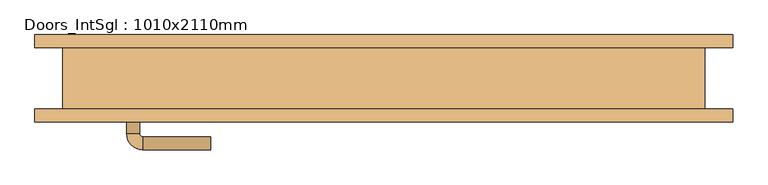
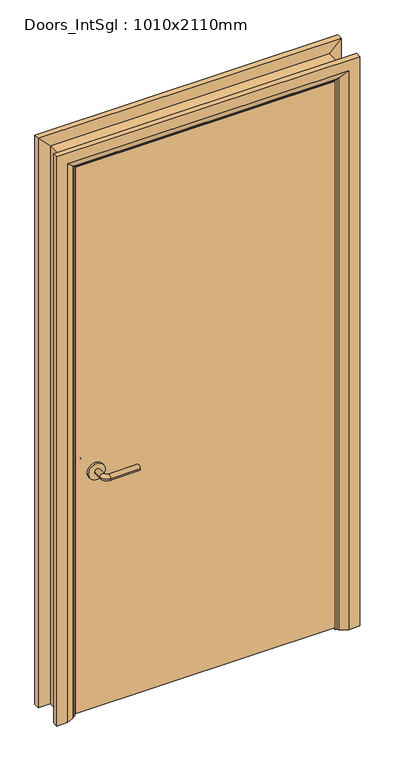
"""IFC4 building model written with IfcOpenShell, lengths in millimetres: door geometry, Doors_IntSgl : 1010x2110mm."""

import ifcopenshell
import ifcopenshell.guid

model = None  # the IFC model being written
_history = None  # IfcOwnerHistory: only IFC2X3 demands one
_inside = {}  # id of a spatial element -> (the spatial element, [elements in it])
_under = {}  # id of a project, library or spatial element -> (it, [spatial elements below it])
_declared = {}  # id of a project -> (the project, [libraries it declares])
_typed = {}  # id of a type object -> (the type object, [elements of that type])
_made_of = {}  # id of a material, layer set ... -> (it, [elements and type objects made of it])


def new_model(schema):
    """Start an empty IFC model of exactly this schema.

    Asked for "IFC4X3", IfcOpenShell would pick the latest addendum, in which some entities
    have other attributes; the version numbers below select the first issue.
    IFC2X3 requires an IfcOwnerHistory on every rooted entity: one is made here for all.
    """
    global model, _history
    if schema == "IFC4X3":
        model = ifcopenshell.file(schema_version=(4, 3, 0, 0))
    else:
        model = ifcopenshell.file(schema=schema)
    _inside.clear()
    _under.clear()
    _declared.clear()
    _typed.clear()
    _made_of.clear()
    _history = None
    if model.schema == "IFC2X3":
        org = make("IfcOrganization", Name="unknown")
        user = make(
            "IfcPersonAndOrganization",
            ThePerson=make("IfcPerson", FamilyName="unknown"),
            TheOrganization=org,
        )
        app = make(
            "IfcApplication",
            ApplicationDeveloper=org,
            Version="unknown",
            ApplicationFullName="unknown",
            ApplicationIdentifier="unknown",
        )
        _history = make(
            "IfcOwnerHistory",
            OwningUser=user,
            OwningApplication=app,
            ChangeAction="ADDED",
            CreationDate=0,
        )
    return model


def make(cls, **values):
    """One entity of the class cls with the attributes given. An attribute that is None is left unset."""
    return model.create_entity(
        cls, **{name: value for name, value in values.items() if value is not None}
    )


def rooted(cls, **values):
    """An entity with a GlobalId (a new one), such as an element, a storey or a relation."""
    return make(cls, GlobalId=ifcopenshell.guid.new(), OwnerHistory=_history, **values)


def si_unit(unit_type, name, prefix=None):
    """IfcSIUnit, for example si_unit("LENGTHUNIT", "METRE", prefix="MILLI")."""
    return make("IfcSIUnit", UnitType=unit_type, Prefix=prefix, Name=name)


def assignment(units):
    """IfcUnitAssignment: the units of a project."""
    return None if units is None else make("IfcUnitAssignment", Units=units)


def point(xyz):
    """IfcCartesianPoint."""
    return None if xyz is None else make("IfcCartesianPoint", Coordinates=xyz)


def direction(xyz):
    """IfcDirection."""
    return None if xyz is None else make("IfcDirection", DirectionRatios=xyz)


def frame(location, z_axis=None, x_axis=None):
    """IfcAxis2Placement3D, a coordinate frame: its origin and axes. An axis left out is left unset."""
    return make(
        "IfcAxis2Placement3D",
        Location=point(location),
        Axis=direction(z_axis),
        RefDirection=direction(x_axis),
    )


def frame_2d(location, x_axis=None):
    """IfcAxis2Placement2D, a coordinate frame in the plane: its origin and x axis."""
    return make(
        "IfcAxis2Placement2D", Location=point(location), RefDirection=direction(x_axis)
    )


def origin():
    """The frame at (0, 0, 0) with its axes left unset."""
    return frame((0.0, 0.0, 0.0))


def place(relative_to, where):
    """IfcLocalPlacement: puts the frame where relative to a parent placement (None: the world)."""
    return make(
        "IfcLocalPlacement", PlacementRelTo=relative_to, RelativePlacement=where
    )


def context(
    kind, dimensions, precision=None, world=None, true_north=None, identifier=None
):
    """IfcGeometricRepresentationContext, for example the 3D "Model" context."""
    return make(
        "IfcGeometricRepresentationContext",
        ContextIdentifier=identifier,
        ContextType=kind,
        CoordinateSpaceDimension=dimensions,
        Precision=precision,
        WorldCoordinateSystem=world,
        TrueNorth=true_north,
    )


def project(units=None, contexts=None):
    """IfcProject with its units and contexts."""
    return rooted(
        "IfcProject",
        Name="project",
        RepresentationContexts=contexts,
        UnitsInContext=assignment(units),
    )


def spatial(cls, under=None, at=None, **own):
    """A site, building, storey or space (cls), placed at a placement, below another one or the project."""
    s = rooted(cls, ObjectPlacement=at, **own)
    if under is not None:
        _under.setdefault(under.id(), (under, []))[1].append(s)
    return s


def polyline(points):
    """IfcPolyline through the points."""
    return make("IfcPolyline", Points=[point(p) for p in points])


def circle_curve(where, radius):
    """IfcCircle in the frame where."""
    return make("IfcCircle", Position=where, Radius=radius)


def ellipse_curve(where, semi_axis1, semi_axis2):
    """IfcEllipse in the frame where."""
    return make(
        "IfcEllipse", Position=where, SemiAxis1=semi_axis1, SemiAxis2=semi_axis2
    )


def trimmed(basis, trim1, trim2, sense, master):
    """IfcTrimmedCurve: the piece of a basis curve between two trims."""
    return make(
        "IfcTrimmedCurve",
        BasisCurve=basis,
        Trim1=trim1,
        Trim2=trim2,
        SenseAgreement=sense,
        MasterRepresentation=master,
    )


def segment(curve, same_sense, transition):
    """IfcCompositeCurveSegment."""
    return make(
        "IfcCompositeCurveSegment",
        Transition=transition,
        SameSense=same_sense,
        ParentCurve=curve,
    )


def composite_curve(segments, self_intersect=None):
    """IfcCompositeCurve: segments joined end to end."""
    return make("IfcCompositeCurve", Segments=segments, SelfIntersect=self_intersect)


def outline(outer, holes=None, kind="AREA"):
    """IfcArbitraryClosedProfileDef: a profile drawn as a closed curve; with holes, ...WithVoids."""
    if holes is None:
        return make("IfcArbitraryClosedProfileDef", ProfileType=kind, OuterCurve=outer)
    return make(
        "IfcArbitraryProfileDefWithVoids",
        ProfileType=kind,
        OuterCurve=outer,
        InnerCurves=holes,
    )


def extrude(swept, where, along, depth):
    """IfcExtrudedAreaSolid: the profile swept, set in the frame where, extruded along a direction by depth."""
    return make(
        "IfcExtrudedAreaSolid",
        SweptArea=swept,
        Position=where,
        ExtrudedDirection=direction(along),
        Depth=depth,
    )


def faces_of(points, faces, orient=None, outer=None):
    """IfcFace entities. A face is a list of loops; a loop is a list of indices into points, from 0.

    orient and outer hold one flag for each loop. By default every Orientation is true, the
    first loop of a face is its IfcFaceOuterBound and the others are IfcFaceBound.
    """
    made = []
    for i, loops in enumerate(faces):
        bounds = []
        for j, loop in enumerate(loops):
            is_outer = j == 0 if outer is None else outer[i][j]
            bounds.append(
                make(
                    "IfcFaceOuterBound" if is_outer else "IfcFaceBound",
                    Bound=make("IfcPolyLoop", Polygon=[points[k] for k in loop]),
                    Orientation=True if orient is None else orient[i][j],
                )
            )
        made.append(make("IfcFace", Bounds=bounds))
    return made


def faceted_brep(points, faces, orient=None, outer=None, voids=None):
    """IfcFacetedBrep: a solid bounded by flat faces; with voids (closed shells), ...WithVoids."""
    shared = [point(p) for p in points]
    hull = make("IfcClosedShell", CfsFaces=faces_of(shared, faces, orient, outer))
    if voids is None:
        return make("IfcFacetedBrep", Outer=hull)
    return make(
        "IfcFacetedBrepWithVoids",
        Outer=hull,
        Voids=[
            make(cls, CfsFaces=faces_of(shared, fs, o, b)) for cls, fs, o, b in voids
        ],
    )


def shape(context_of_items, identifier, shape_type, items):
    """IfcShapeRepresentation: the items that make up one representation, for example the "Body"."""
    return make(
        "IfcShapeRepresentation",
        ContextOfItems=context_of_items,
        RepresentationIdentifier=identifier,
        RepresentationType=shape_type,
        Items=items,
    )


def source(mapping_origin, context_of_items, identifier, shape_type, items):
    """IfcRepresentationMap: a shape defined once, which mapped items show again and again."""
    return make(
        "IfcRepresentationMap",
        MappingOrigin=mapping_origin,
        MappedRepresentation=shape(context_of_items, identifier, shape_type, items),
    )


def transform(
    local_origin,
    x_axis=None,
    y_axis=None,
    z_axis=None,
    scale=None,
    scale2=None,
    scale3=None,
    uniform=True,
):
    """IfcCartesianTransformationOperator3D, or its non-uniform kind. x_axis, y_axis, z_axis: its Axis1, 2, 3."""
    if uniform:
        return make(
            "IfcCartesianTransformationOperator3D",
            Axis1=direction(x_axis),
            Axis2=direction(y_axis),
            LocalOrigin=point(local_origin),
            Scale=scale,
            Axis3=direction(z_axis),
        )
    return make(
        "IfcCartesianTransformationOperator3DnonUniform",
        Axis1=direction(x_axis),
        Axis2=direction(y_axis),
        LocalOrigin=point(local_origin),
        Scale=scale,
        Axis3=direction(z_axis),
        Scale2=scale2,
        Scale3=scale3,
    )


def mapped(mapping_source, mapping_target):
    """IfcMappedItem: shows the shape of a source again, moved by a transform."""
    return make(
        "IfcMappedItem", MappingSource=mapping_source, MappingTarget=mapping_target
    )


def made_of(thing, what):
    """Note that an element or type object is made of a material, layer set ...; save() writes the relation."""
    if what is not None:
        _made_of.setdefault(what.id(), (what, []))[1].append(thing)
    return thing


def element(
    cls,
    number,
    at=None,
    inside=None,
    cuts=None,
    type_object=None,
    material=None,
    context=None,
    identifier="Body",
    shape_type=None,
    held_by="IfcProductDefinitionShape",
    body=None,
    shapes=None,
    **own,
):
    """One element of the class cls, such as IfcWall. Its Tag is "e" and its number.

    at: its placement. inside: the storey or other place that contains it. cuts: it is an
    opening in that element (IfcRelVoidsElement). A single representation is given by context,
    identifier, shape_type and body (its items); several are given by shapes. held_by: the class
    of the entity that holds the representations. save() writes the other relations.
    """
    e = rooted(cls, Tag="e%d" % number, ObjectPlacement=at, **own)
    if body is not None:
        shapes = [shape(context, identifier, shape_type, body)]
    if shapes is not None:
        e.Representation = make(held_by, Representations=shapes)
    if inside is not None:
        _inside.setdefault(inside.id(), (inside, []))[1].append(e)
    if cuts is not None:
        rooted(
            "IfcRelVoidsElement", RelatingBuildingElement=cuts, RelatedOpeningElement=e
        )
    if type_object is not None:
        _typed.setdefault(type_object.id(), (type_object, []))[1].append(e)
    return made_of(e, material)


def aggregate(whole, parts):
    """IfcRelAggregates: a whole, such as a stair, and the parts it consists of."""
    return rooted("IfcRelAggregates", RelatingObject=whole, RelatedObjects=parts)


def save(model, path):
    """Write the relations noted so far, then the file.

    IfcRelAggregates (storeys below a building ...), IfcRelContainedInSpatialStructure (elements
    in a storey), IfcRelDefinesByType, IfcRelAssociatesMaterial and IfcRelDeclares: one each for
    every whole, place, type object, material and project.
    """
    for whole, parts in _under.values():
        aggregate(whole, parts)
    for where, things in _inside.values():
        rooted(
            "IfcRelContainedInSpatialStructure",
            RelatedElements=things,
            RelatingStructure=where,
        )
    for kind, things in _typed.values():
        rooted("IfcRelDefinesByType", RelatedObjects=things, RelatingType=kind)
    for what, things in _made_of.values():
        rooted("IfcRelAssociatesMaterial", RelatedObjects=things, RelatingMaterial=what)
    for by, libraries in _declared.values():
        rooted("IfcRelDeclares", RelatingContext=by, RelatedDefinitions=libraries)
    model.write(path)


def plane_surface(at):
    """IfcPlane: the flat surface through the origin of the frame at, square to its z axis."""
    return make("IfcPlane", Position=at)


def cylinder_surface(at, radius):
    """IfcCylindricalSurface: all points at the distance radius from the z axis of the frame at."""
    return make("IfcCylindricalSurface", Position=at, Radius=radius)


def revolved_surface(curve, axis_point, axis_direction):
    """IfcSurfaceOfRevolution: the curve turned about the line through axis_point along axis_direction."""
    return make(
        "IfcSurfaceOfRevolution",
        SweptCurve=make("IfcArbitraryOpenProfileDef", ProfileType="CURVE", Curve=curve),
        AxisPosition=make("IfcAxis1Placement", Location=point(axis_point), Axis=direction(axis_direction)),
    )


def advanced_brep(points, edges, surfaces, faces):
    """IfcAdvancedBrep: a solid bounded by faces that lie on surfaces and meet in shared edges.

    An edge is (start, end): straight between two places in points (the first is 0);
    or (start, end, curve); or (start, end, curve, False) where it runs against its curve.
    A face is (place in surfaces, loops), or (place, loops, False) where it looks against
    its surface's normal. A loop lists edges by number (the first is 1), with a minus sign
    where the edge is run from its end to its start. The first loop is the outer one.
    """
    corners = [point(p) for p in points]
    vertices = [make("IfcVertexPoint", VertexGeometry=c) for c in corners]
    made = []
    for start, end, *more in edges:
        made.append(
            make(
                "IfcEdgeCurve",
                EdgeStart=vertices[start],
                EdgeEnd=vertices[end],
                EdgeGeometry=more[0] if more else make("IfcPolyline", Points=[corners[start], corners[end]]),
                SameSense=more[1] if len(more) > 1 else True,
            )
        )
    hull = []
    for where, loops, *sense in faces:
        bounds = []
        for j, loop in enumerate(loops):
            ring = [make("IfcOrientedEdge", EdgeElement=made[abs(k) - 1], Orientation=k > 0) for k in loop]
            bounds.append(
                make(
                    "IfcFaceOuterBound" if j == 0 else "IfcFaceBound",
                    Bound=make("IfcEdgeLoop", EdgeList=ring),
                    Orientation=True,
                )
            )
        hull.append(make("IfcAdvancedFace", Bounds=bounds, FaceSurface=surfaces[where], SameSense=sense[0] if sense else True))
    return make("IfcAdvancedBrep", Outer=make("IfcClosedShell", CfsFaces=hull))


def doors_intsgl_1010x2110mm_25c8a350(model_context):
    return source(origin(), model_context, "Body", "SolidModel", [
        advanced_brep(
        [(-398.0, -1.5, 900.0), (-378.0, -1.5, 900.0), (-398.0, 28.5, 900.0), (-378.0, 28.5, 900.0), (-373.0, 33.5, 900.0), (-373.0, 53.5, 900.0), (-268.0, 53.5, 900.0), (-268.0, 33.5, 900.0)],
        [
            (0, 1, circle_curve(frame((-388.0, -1.5, 900.0), z_axis=(0.0, -1.0, 0.0), x_axis=(1.0, 0.0, 0.0)), 10.0)),
            (1, 0, circle_curve(frame((-388.0, -1.5, 900.0), z_axis=(0.0, -1.0, 0.0), x_axis=(1.0, 0.0, 0.0)), 10.0)),
            (0, 2),
            (2, 3, circle_curve(frame((-388.0, 28.5, 900.0), z_axis=(0.0, -1.0, 0.0), x_axis=(1.0, 0.0, 0.0)), 10.0)),
            (3, 1),
            (3, 2, circle_curve(frame((-388.0, 28.5, 900.0), z_axis=(0.0, -1.0, 0.0), x_axis=(1.0, 0.0, 0.0)), 10.0)),
            (4, 3, circle_curve(frame((-373.0, 28.5, 900.0), z_axis=(0.0, 0.0, 1.0), x_axis=(-1.0, 0.0, 0.0)), 5.0)),
            (2, 5, circle_curve(frame((-373.0, 28.5, 900.0), z_axis=(0.0, 0.0, -1.0), x_axis=(-1.0, 0.0, 0.0)), 25.0)),
            (5, 4, circle_curve(frame((-373.0, 43.5, 900.0), z_axis=(-1.0, 0.0, 0.0), x_axis=(0.0, -1.0, 0.0)), 10.0)),
            (4, 5, circle_curve(frame((-373.0, 43.5, 900.0), z_axis=(-1.0, 0.0, 0.0), x_axis=(0.0, -1.0, 0.0)), 10.0)),
            (6, 7, circle_curve(frame((-268.0, 43.5, 900.0), z_axis=(1.0, 0.0, 0.0), x_axis=(0.0, -1.0, 0.0)), 10.0)),
            (7, 6, circle_curve(frame((-268.0, 43.5, 900.0), z_axis=(1.0, 0.0, 0.0), x_axis=(0.0, -1.0, 0.0)), 10.0)),
            (5, 6),
            (7, 4),
        ],
        [
            plane_surface(frame((-388.0, -1.5, 900.0), z_axis=(0.0, -1.0, 0.0), x_axis=(0.0, 0.0, 1.0))),
            cylinder_surface(frame((-388.0, -1.5, 900.0), z_axis=(0.0, -1.0, 0.0), x_axis=(1.0, 0.0, 0.0)), 10.0),
            revolved_surface(trimmed(ellipse_curve(frame((-388.0, 28.5, 900.0), z_axis=(0.0, -1.0, 0.0), x_axis=(1.0, 0.0, 0.0)), 10.0, 10.0), [point((-398.0, 28.5, 900.0))], [point((-378.0, 28.5, 900.0))], True, "CARTESIAN"), (-373.0, 28.5, 900.0), (0.0, 0.0, -1.0)),
            revolved_surface(trimmed(ellipse_curve(frame((-388.0, 28.5, 900.0), z_axis=(0.0, -1.0, 0.0), x_axis=(1.0, 0.0, 0.0)), 10.0, 10.0), [point((-378.0, 28.5, 900.0))], [point((-398.0, 28.5, 900.0))], True, "CARTESIAN"), (-373.0, 28.5, 900.0), (0.0, 0.0, -1.0)),
            plane_surface(frame((-268.0, 43.5, 900.0), z_axis=(1.0, 0.0, 0.0), x_axis=(0.0, 0.0, 1.0))),
            cylinder_surface(frame((-373.0, 43.5, 900.0), z_axis=(-1.0, 0.0, 0.0), x_axis=(0.0, -1.0, 0.0)), 10.0),
        ],
        [
            (0, [[1, 2]]),
            (1, [[-1, 3, 4, 5]]),
            (1, [[-2, -5, 6, -3]]),
            (2, [[7, -4, 8, 9]]),
            (3, [[-8, -6, -7, 10]]),
            (4, [[11, 12]]),
            (5, [[-9, 13, -12, 14]]),
            (5, [[-10, -14, -11, -13]]),
        ],
    ),
        extrude(outline(composite_curve([segment(trimmed(circle_curve(frame_2d((900.0, -390.5)), 30.0), [point((900.0, -420.5))], [point((900.0, -360.5))], False, "CARTESIAN"), True, "CONTINUOUS"), segment(trimmed(circle_curve(frame_2d((900.0, -390.5)), 30.0), [point((900.0, -360.5))], [point((900.0, -420.5))], False, "CARTESIAN"), True, "CONTINUOUS")], self_intersect=False)), frame((0.0, -9.5, 0.0), z_axis=(0.0, 1.0, 0.0), x_axis=(0.0, 0.0, 1.0)), (0.0, 0.0, 1.0), 8.0),
        advanced_brep(
        [(-398.0, -55.5, 900.0), (-378.0, -55.5, 900.0), (-378.0, -85.5, 900.0), (-398.0, -85.5, 900.0), (-373.0, -90.5, 900.0), (-373.0, -110.5, 900.0), (-268.0, -110.5, 900.0), (-268.0, -90.5, 900.0)],
        [
            (0, 1, circle_curve(frame((-388.0, -55.5, 900.0), z_axis=(0.0, 1.0, 0.0), x_axis=(1.0, 0.0, 0.0)), 10.0)),
            (1, 0, circle_curve(frame((-388.0, -55.5, 900.0), z_axis=(0.0, 1.0, 0.0), x_axis=(1.0, 0.0, 0.0)), 10.0)),
            (1, 2),
            (2, 3, circle_curve(frame((-388.0, -85.5, 900.0), z_axis=(0.0, 1.0, 0.0), x_axis=(1.0, 0.0, 0.0)), 10.0)),
            (3, 0),
            (3, 2, circle_curve(frame((-388.0, -85.5, 900.0), z_axis=(0.0, 1.0, 0.0), x_axis=(1.0, 0.0, 0.0)), 10.0)),
            (4, 5, circle_curve(frame((-373.0, -100.5, 900.0), z_axis=(-1.0, 0.0, 0.0), x_axis=(0.0, 1.0, 0.0)), 10.0)),
            (5, 3, circle_curve(frame((-373.0, -85.5, 900.0), z_axis=(0.0, 0.0, -1.0), x_axis=(-1.0, 0.0, 0.0)), 25.0)),
            (2, 4, circle_curve(frame((-373.0, -85.5, 900.0), z_axis=(0.0, 0.0, 1.0), x_axis=(-1.0, 0.0, 0.0)), 5.0)),
            (5, 4, circle_curve(frame((-373.0, -100.5, 900.0), z_axis=(-1.0, 0.0, 0.0), x_axis=(0.0, 1.0, 0.0)), 10.0)),
            (6, 7, circle_curve(frame((-268.0, -100.5, 900.0), z_axis=(1.0, 0.0, 0.0), x_axis=(0.0, 1.0, 0.0)), 10.0)),
            (7, 6, circle_curve(frame((-268.0, -100.5, 900.0), z_axis=(1.0, 0.0, 0.0), x_axis=(0.0, 1.0, 0.0)), 10.0)),
            (4, 7),
            (6, 5),
        ],
        [
            plane_surface(frame((-388.0, -55.5, 900.0), z_axis=(0.0, 1.0, 0.0), x_axis=(0.0, 0.0, 1.0))),
            cylinder_surface(frame((-388.0, -55.5, 900.0), z_axis=(0.0, 1.0, 0.0), x_axis=(1.0, 0.0, 0.0)), 10.0),
            revolved_surface(trimmed(ellipse_curve(frame((-388.0, -85.5, 900.0), z_axis=(0.0, -1.0, 0.0), x_axis=(1.0, 0.0, 0.0)), 10.0, 10.0), [point((-398.0, -85.5, 900.0))], [point((-378.0, -85.5, 900.0))], True, "CARTESIAN"), (-373.0, -85.5, 900.0), (0.0, 0.0, -1.0)),
            revolved_surface(trimmed(ellipse_curve(frame((-388.0, -85.5, 900.0), z_axis=(0.0, -1.0, 0.0), x_axis=(1.0, 0.0, 0.0)), 10.0, 10.0), [point((-378.0, -85.5, 900.0))], [point((-398.0, -85.5, 900.0))], True, "CARTESIAN"), (-373.0, -85.5, 900.0), (0.0, 0.0, -1.0)),
            plane_surface(frame((-268.0, -100.5, 900.0), z_axis=(1.0, 0.0, 0.0), x_axis=(0.0, 0.0, 1.0))),
            cylinder_surface(frame((-373.0, -100.5, 900.0), z_axis=(-1.0, 0.0, 0.0), x_axis=(0.0, 1.0, 0.0)), 10.0),
        ],
        [
            (0, [[1, 2]]),
            (1, [[3, 4, 5, -2]]),
            (1, [[-5, 6, -3, -1]]),
            (2, [[7, 8, -4, 9]]),
            (3, [[10, -9, -6, -8]]),
            (4, [[11, 12]]),
            (5, [[13, -11, 14, -7]]),
            (5, [[-14, -12, -13, -10]]),
        ],
    ),
        extrude(outline(composite_curve([segment(trimmed(circle_curve(frame_2d((900.0, -390.5)), 30.0), [point((900.0, -420.5))], [point((900.0, -360.5))], False, "CARTESIAN"), True, "CONTINUOUS"), segment(trimmed(circle_curve(frame_2d((900.0, -390.5)), 30.0), [point((900.0, -360.5))], [point((900.0, -420.5))], False, "CARTESIAN"), True, "CONTINUOUS")], self_intersect=False)), frame((0.0, -55.5, 0.0), z_axis=(0.0, 1.0, 0.0), x_axis=(0.0, 0.0, 1.0)), (0.0, 0.0, 1.0), 8.0),
        extrude(outline(polyline([(463.0, -9.5), (463.0, -47.5), (-463.0, -47.5), (-463.0, -9.5), (463.0, -9.5)])), frame((0.0, 0.0, 8.0), z_axis=(0.0, 0.0, 1.0), x_axis=(1.0, 0.0, 0.0)), (0.0, 0.0, 1.0), 2060.0),
        advanced_brep(
        [(540.0, -67.5, 0.0), (500.0, -67.5, 0.0), (474.0, -53.5, 0.0), (470.0, -47.5, 0.0), (540.0, -47.5, 0.0), (540.0, -47.5, 2145.0), (540.0, -67.5, 2145.0), (470.0, -47.5, 2075.0), (-470.0, -47.5, 2075.0), (-470.0, -47.5, 0.0), (-540.0, -47.5, 0.0), (-540.0, -47.5, 2145.0), (474.0, -53.5, 2079.0), (500.0, -67.5, 2105.0), (-540.0, -67.5, 2145.0), (-540.0, -67.5, 0.0), (-500.0, -67.5, 0.0), (-500.0, -67.5, 2105.0), (-474.0, -53.5, 2079.0), (-474.0, -53.5, 0.0)],
        [
            (0, 1),
            (1, 2),
            (2, 3, circle_curve(frame((478.0, -46.5, 0.0), z_axis=(0.0, 0.0, -1.0), x_axis=(1.0, 0.0, 0.0)), 8.0622577)),
            (3, 4),
            (4, 0),
            (4, 5),
            (5, 6),
            (6, 0),
            (3, 7),
            (7, 8),
            (8, 9),
            (9, 10),
            (10, 11),
            (11, 5),
            (2, 12),
            (12, 7, ellipse_curve(frame((478.0, -46.5, 2083.0), z_axis=(0.7071067811865475, 0.0, -0.7071067811865475), x_axis=(-0.7071067811865474, 0.0, -0.7071067811865476)), 11.4017543, 8.0622577)),
            (1, 13),
            (13, 12),
            (6, 14),
            (14, 15),
            (15, 16),
            (16, 17),
            (17, 13),
            (11, 14),
            (12, 18),
            (18, 8, ellipse_curve(frame((-478.0, -46.5, 2083.0), z_axis=(0.7071067811865475, 0.0, 0.7071067811865475), x_axis=(0.7071067811865476, 0.0, -0.7071067811865474)), 11.4017543, 8.0622577)),
            (17, 18),
            (15, 10),
            (9, 19, circle_curve(frame((-478.0, -46.5, 0.0), z_axis=(0.0, 0.0, -1.0), x_axis=(-1.0, 0.0, 0.0)), 8.0622577)),
            (19, 16),
            (18, 19),
        ],
        [
            plane_surface(frame((470.0, -47.5, 0.0), z_axis=(0.0, 0.0, -1.0), x_axis=(0.0, 1.0, 0.0))),
            plane_surface(frame((540.0, -67.5, 0.0), z_axis=(1.0, 0.0, 0.0), x_axis=(0.0, 0.0, 1.0))),
            plane_surface(frame((540.0, -47.5, 0.0), z_axis=(0.0, 1.0, 0.0), x_axis=(0.0, 0.0, 1.0))),
            cylinder_surface(frame((478.0, -46.5, 0.0), z_axis=(0.0, 0.0, -1.0), x_axis=(1.0, 0.0, 0.0)), 8.0622577),
            plane_surface(frame((474.0, -53.5, 0.0), z_axis=(-0.4740998230350126, -0.880471099922178, 0.0), x_axis=(0.0, 0.0, 1.0))),
            plane_surface(frame((500.0, -67.5, 0.0), z_axis=(0.0, -1.0, 0.0), x_axis=(0.0, 0.0, 1.0))),
            plane_surface(frame((540.0, -67.5, 2145.0), z_axis=(0.0, 0.0, 1.0), x_axis=(-1.0, 0.0, 0.0))),
            cylinder_surface(frame((470.0, -46.5, 2083.0), z_axis=(1.0, 0.0, 0.0), x_axis=(0.0, 0.0, 1.0)), 8.0622577),
            plane_surface(frame((474.0, -53.5, 2079.0), z_axis=(0.0, -0.8804710999221764, -0.4740998230350154), x_axis=(-1.0, 0.0, 0.0))),
            plane_surface(frame((-470.0, -47.5, 0.0), z_axis=(0.0, 0.0, -1.0), x_axis=(0.0, 1.0, 0.0))),
            plane_surface(frame((-540.0, -67.5, 2145.0), z_axis=(-1.0, 0.0, 0.0), x_axis=(0.0, 0.0, -1.0))),
            cylinder_surface(frame((-478.0, -46.5, 2075.0), z_axis=(0.0, 0.0, 1.0), x_axis=(-1.0, 0.0, 0.0)), 8.0622577),
            plane_surface(frame((-474.0, -53.5, 2079.0), z_axis=(0.47409982303501824, -0.8804710999221749, 0.0), x_axis=(0.0, 0.0, -1.0))),
        ],
        [
            (0, [[1, 2, 3, 4, 5]]),
            (1, [[6, 7, 8, -5]]),
            (2, [[9, 10, 11, 12, 13, 14, -6, -4]]),
            (3, [[15, 16, -9, -3]]),
            (4, [[17, 18, -15, -2]]),
            (5, [[-8, 19, 20, 21, 22, 23, -17, -1]]),
            (6, [[-14, 24, -19, -7]]),
            (7, [[25, 26, -10, -16]]),
            (8, [[-23, 27, -25, -18]]),
            (9, [[28, -12, 29, 30, -21]]),
            (10, [[-13, -28, -20, -24]]),
            (11, [[31, -29, -11, -26]]),
            (12, [[-22, -30, -31, -27]]),
        ],
    ),
        extrude(outline(polyline([(0.0, -446.0), (2051.0, -446.0), (2051.0, 446.0), (0.0, 446.0), (0.0, 465.0), (2070.0, 465.0), (2070.0, -465.0), (0.0, -465.0), (0.0, -446.0)])), frame((0.0, -7.5, 0.0), z_axis=(0.0, 1.0, 0.0), x_axis=(0.0, 0.0, 1.0)), (0.0, 0.0, 1.0), 32.0),
        advanced_brep(
        [(-540.0, 67.5, 0.0), (-500.0, 67.5, 0.0), (-474.0, 53.5, 0.0), (-470.0, 47.5, 0.0), (-540.0, 47.5, 0.0), (-540.0, 47.5, 2145.0), (-540.0, 67.5, 2145.0), (-470.0, 47.5, 2075.0), (-474.0, 53.5, 2079.0), (-500.0, 67.5, 2105.0), (540.0, 47.5, 2145.0), (540.0, 67.5, 2145.0), (470.0, 47.5, 2075.0), (474.0, 53.5, 2079.0), (500.0, 67.5, 2105.0), (540.0, 67.5, 0.0), (540.0, 47.5, 0.0), (470.0, 47.5, 0.0), (474.0, 53.5, 0.0), (500.0, 67.5, 0.0)],
        [
            (0, 1),
            (1, 2),
            (2, 3, circle_curve(frame((-478.0, 46.5, 0.0), z_axis=(0.0, 0.0, -1.0), x_axis=(-1.0, 0.0, 0.0)), 8.0622577)),
            (3, 4),
            (4, 0),
            (4, 5),
            (5, 6),
            (6, 0),
            (3, 7),
            (7, 5),
            (2, 8),
            (8, 7, ellipse_curve(frame((-478.0, 46.5, 2083.0), z_axis=(-0.7071067811865475, 0.0, -0.7071067811865475), x_axis=(0.7071067811865474, 0.0, -0.7071067811865476)), 11.4017543, 8.0622577)),
            (1, 9),
            (9, 8),
            (6, 9),
            (5, 10),
            (10, 11),
            (11, 6),
            (7, 12),
            (12, 10),
            (8, 13),
            (13, 12, ellipse_curve(frame((478.0, 46.5, 2083.0), z_axis=(-0.7071067811865475, 0.0, 0.7071067811865475), x_axis=(-0.7071067811865476, 0.0, -0.7071067811865474)), 11.4017543, 8.0622577)),
            (9, 14),
            (14, 13),
            (11, 14),
            (15, 16),
            (16, 17),
            (17, 18, circle_curve(frame((478.0, 46.5, 0.0), z_axis=(0.0, 0.0, -1.0), x_axis=(1.0, 0.0, 0.0)), 8.0622577)),
            (18, 19),
            (19, 15),
            (10, 16),
            (15, 11),
            (12, 17),
            (13, 18),
            (14, 19),
        ],
        [
            plane_surface(frame((-470.0, 120.3010989, 0.0), z_axis=(0.0, 0.0, -1.0), x_axis=(1.0, 0.0, 0.0))),
            plane_surface(frame((-540.0, 67.5, 0.0), z_axis=(-1.0, 0.0, 0.0), x_axis=(0.0, 0.0, 1.0))),
            plane_surface(frame((-540.0, 47.5, 0.0), z_axis=(0.0, -1.0, 0.0), x_axis=(0.0, 0.0, 1.0))),
            cylinder_surface(frame((-478.0, 46.5, 0.0), z_axis=(0.0, 0.0, -1.0), x_axis=(-1.0, 0.0, 0.0)), 8.0622577),
            plane_surface(frame((-474.0, 53.5, 0.0), z_axis=(0.4740998230350183, 0.8804710999221749, 0.0), x_axis=(0.0, 0.0, 1.0))),
            plane_surface(frame((-500.0, 67.5, 0.0), z_axis=(0.0, 1.0, 0.0), x_axis=(0.0, 0.0, 1.0))),
            plane_surface(frame((-540.0, 67.5, 2145.0), z_axis=(0.0, 0.0, 1.0), x_axis=(1.0, 0.0, 0.0))),
            plane_surface(frame((-540.0, 47.5, 2145.0), z_axis=(0.0, -1.0, 0.0), x_axis=(1.0, 0.0, 0.0))),
            cylinder_surface(frame((-470.0, 46.5, 2083.0), z_axis=(-1.0, 0.0, 0.0), x_axis=(0.0, 0.0, 1.0)), 8.0622577),
            plane_surface(frame((-474.0, 53.5, 2079.0), z_axis=(0.0, 0.8804710999221749, -0.4740998230350183), x_axis=(1.0, 0.0, 0.0))),
            plane_surface(frame((-500.0, 67.5, 2105.0), z_axis=(0.0, 1.0, 0.0), x_axis=(1.0, 0.0, 0.0))),
            plane_surface(frame((470.0, 120.3010989, 0.0), z_axis=(0.0, 0.0, -1.0), x_axis=(-1.0, 0.0, 0.0))),
            plane_surface(frame((540.0, 67.5, 2145.0), z_axis=(1.0, 0.0, 0.0), x_axis=(0.0, 0.0, -1.0))),
            plane_surface(frame((540.0, 47.5, 2145.0), z_axis=(0.0, -1.0, 0.0), x_axis=(0.0, 0.0, -1.0))),
            cylinder_surface(frame((478.0, 46.5, 2075.0), z_axis=(0.0, 0.0, 1.0), x_axis=(1.0, 0.0, 0.0)), 8.0622577),
            plane_surface(frame((474.0, 53.5, 2079.0), z_axis=(-0.4740998230350183, 0.8804710999221749, 0.0), x_axis=(0.0, 0.0, -1.0))),
            plane_surface(frame((500.0, 67.5, 2105.0), z_axis=(0.0, 1.0, 0.0), x_axis=(0.0, 0.0, -1.0))),
        ],
        [
            (0, [[1, 2, 3, 4, 5]]),
            (1, [[6, 7, 8, -5]]),
            (2, [[9, 10, -6, -4]]),
            (3, [[11, 12, -9, -3]]),
            (4, [[13, 14, -11, -2]]),
            (5, [[-8, 15, -13, -1]]),
            (6, [[16, 17, 18, -7]]),
            (7, [[19, 20, -16, -10]]),
            (8, [[21, 22, -19, -12]]),
            (9, [[23, 24, -21, -14]]),
            (10, [[-18, 25, -23, -15]]),
            (11, [[26, 27, 28, 29, 30]]),
            (12, [[31, -26, 32, -17]]),
            (13, [[33, -27, -31, -20]]),
            (14, [[34, -28, -33, -22]]),
            (15, [[35, -29, -34, -24]]),
            (16, [[-32, -30, -35, -25]]),
        ],
    ),
        faceted_brep([(-465.0, -47.5, 0.0), (-497.0, -47.5, 0.0), (-497.0, 47.5, 0.0), (-465.0, 47.5, 0.0), (-465.0, 47.5, 2070.0), (-465.0, -47.5, 2070.0), (-497.0, 47.5, 2102.0), (-497.0, -47.5, 2102.0), (465.0, 47.5, 2070.0), (465.0, -47.5, 2070.0), (497.0, 47.5, 2102.0), (497.0, -47.5, 2102.0), (465.0, -47.5, 0.0), (465.0, 47.5, 0.0), (497.0, 47.5, 0.0), (497.0, -47.5, 0.0)], [[[0, 1, 2, 3]], [[3, 4, 5, 0]], [[2, 6, 4, 3]], [[1, 7, 6, 2]], [[0, 5, 7, 1]], [[4, 8, 9, 5]], [[6, 10, 8, 4]], [[7, 11, 10, 6]], [[5, 9, 11, 7]], [[12, 13, 14, 15]], [[8, 13, 12, 9]], [[10, 14, 13, 8]], [[11, 15, 14, 10]], [[9, 12, 15, 11]]]),
    ])


if __name__ == "__main__":
    model = new_model("IFC4")
    model_context = context("Model", 3, world=origin())
    ifc_project = project(units=[si_unit("LENGTHUNIT", "METRE", prefix="MILLI")], contexts=[model_context])
    site = spatial("IfcSite", under=ifc_project)
    building = spatial("IfcBuilding", under=site)
    placement = place(None, origin())
    doors_intsgl_1010x2110mm_shape = doors_intsgl_1010x2110mm_25c8a350(model_context)
    element("IfcDoor", 1, ObjectType="Doors_IntSgl : 1010x2110mm", at=placement, inside=building, context=model_context, shape_type="MappedRepresentation", body=[
        mapped(doors_intsgl_1010x2110mm_shape, transform((0.0, 0.0, 0.0), x_axis=(1.0, 0.0, 0.0), y_axis=(0.0, 1.0, 0.0), z_axis=(0.0, 0.0, 1.0))),
    ])
    save(model, "model.ifc")

# Revit data of these elements
# Type "Doors_IntSgl : 1010x2110mm"
#   Construction Type Id = "MDOOR"
#   Type Mark = "43"
#   Type Comments = "Internal Single"
#   Operation = "SingleSwingRight"
#   Manufacturer = "Revit"
#   Keynote = "L20"
#   Description = "Internal Single Door"
#   Analytic Construction = "Metal"
#   UnderCut = 8 mm
#   Tolerance = 2 mm
#   Thickness = 38 mm
#   Thermal Resistance (R) = 0.270117 (m²·K)/W
#   Structural Tolerance = 8 mm
#   StopDepth = 32 mm
#   Stop Thickness = 19 mm
#   Rough Width = 1010 mm
#   Rough Height = 2110 mm
#   Height to Top Lock Rail = 1000 mm
#   Heat Transfer Coefficient (U) = 3.7021 W/(m²·K)
#   Handle Z Distance = 900 mm
#   Handle X Distance = 75 mm
#   Frame Thickness = 32 mm
#   Door Panel Width = 926 mm
#   Door Panel Thickness = 38 mm
#   Door Panel Offset = 0 mm
#   Height = 2110 mm
#   Width = 1010 mm
#   Door Panel Height = 2060 mm
#   Architrave Setback = 5 mm
#   Vis - Ironmongery = yes
#   Material Ironmongery = Door - Handle
#   Material Frame = Door - Frame/Mullion (1)
#   Material Door = Door - Panel
#   Material Architrave = Door - Architrave
#   Visual Light Transmittance = 0
#   Solar Heat Gain Coefficient = 0
#   Function = (empty or 0)
#   Wall Closure = (empty or 0)
# Element 1 (IfcDoor, "Doors_IntSgl : 1010x2110mm")
#   Materials on its faces: "Door - Architrave", "Door - Handle", "Door - Frame/Mullion (1)", "Door - Panel"
# Materials
#   "Door - Handle": class "Miscellaneous", colour RGB 0 0 0, transparency 0, Keynote = "P21", Cost = 0
#   "Door - Frame/Mullion (1)": class "Wood", colour RGB 212 179 113, transparency 0, Keynote = "L20", Cost = 0
#   "Door - Panel": class "Wood", colour RGB 210 159 95, transparency 0, Keynote = "L20", Cost = 0
#   "Door - Architrave": class "Wood", colour RGB 154 90 5, transparency 0, Keynote = "P20", Cost = 0
